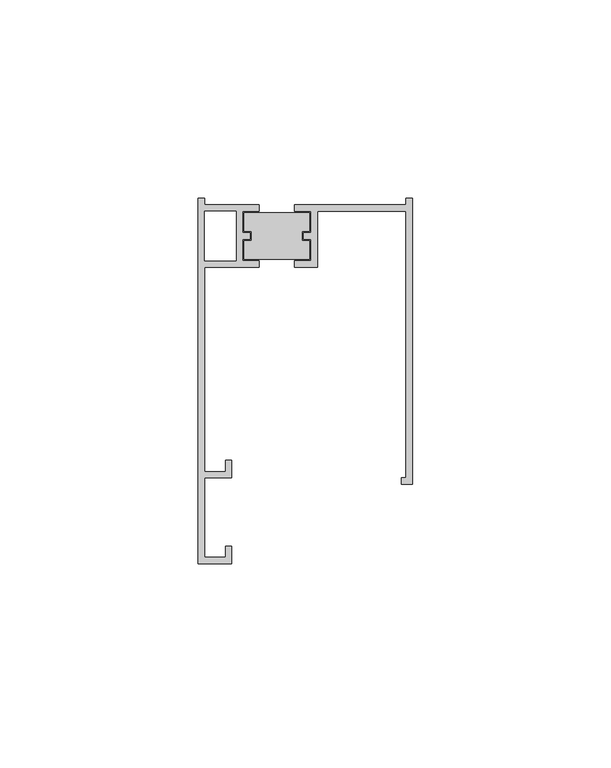
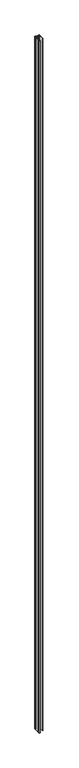
"""IFC4 building model written with IfcOpenShell, lengths in millimetres: proxy geometry, Generic Models 2:Generic Models 2:310765:Generic Models 2:310765 : Generic Models 2:Generic Models 2:310765:15 : Generic Models 2:Generic Models 2:310765:Generic Models 2:310765 : Generic Models 2:Generic Models 2:310765:300385."""

from ifc_helpers import new_model, si_unit, origin, origin_with_axes, place, context, project, spatial, polyline, outline, extrude, source, transform, mapped, element, save


def generic_models_0c4f637a(model_context):
    return source(origin(), model_context, "Body", "SweptSolid", [
        extrude(outline(polyline([(667633.5969099, -670386.8274693), (667617.0446537, -670386.8274693), (667617.0446537, -670382.1299707), (667618.9700691, -670382.1299707), (667618.9700691, -670379.7487207), (667617.0446537, -670379.7487207), (667617.0446537, -670375.0512221), (667633.5969099, -670375.0512221), (667633.5969099, -670379.7487207), (667631.6714944, -670379.7487207), (667631.6714944, -670382.1299707), (667633.5969099, -670382.1299707), (667633.5969099, -670386.8274693)])), origin_with_axes(), (0.0, 0.0, 1.0), 8775.8734497),
        extrude(outline(polyline([(667613.9760152, -670463.4793471), (667605.5296437, -670463.4793471), (667605.5296437, -670371.4793471), (667607.1171437, -670371.4793471), (667607.1171437, -670373.0668471), (667620.8149662, -670373.0668471), (667620.8149662, -670374.6543471), (667616.6477787, -670374.6543471), (667616.6477787, -670380.1455957), (667618.5731941, -670380.1455957), (667618.5731941, -670381.7330957), (667616.6477787, -670381.7330957), (667616.6477787, -670387.2243443), (667620.8149662, -670387.2243443), (667620.8149662, -670388.8118443), (667607.1171437, -670388.8118443), (667607.1171437, -670440.3043471), (667612.3885152, -670440.3043471), (667612.3885152, -670437.5045205), (667613.9760152, -670437.5045205), (667613.9760152, -670441.8918471), (667607.1171437, -670441.8918471), (667607.1171437, -670461.8918471), (667612.3885152, -670461.8918471), (667612.3885152, -670459.0920205), (667613.9760152, -670459.0920205), (667613.9760152, -670463.4793471)]), holes=[polyline([(667607.1171437, -670387.2243443), (667615.0602787, -670387.2243443), (667615.0602787, -670374.6543471), (667607.1171437, -670374.6543471), (667607.1171437, -670387.2243443)])]), origin_with_axes(), (0.0, 0.0, 1.0), 8775.8734497),
        extrude(outline(polyline([(667657.9421437, -670371.4793471), (667659.5296437, -670371.4793471), (667659.5296437, -670443.4793471), (667656.8145537, -670443.4793471), (667656.8145537, -670441.8918471), (667657.9421437, -670441.8918471), (667657.9421437, -670374.6543471), (667635.5812849, -670374.6543471), (667635.5812849, -670388.8118443), (667629.8265974, -670388.8118443), (667629.8265974, -670387.2243443), (667633.9937849, -670387.2243443), (667633.9937849, -670381.7330957), (667632.0683694, -670381.7330957), (667632.0683694, -670380.1455957), (667633.9937849, -670380.1455957), (667633.9937849, -670374.6543471), (667629.8265974, -670374.6543471), (667629.8265974, -670373.0668471), (667657.9421437, -670373.0668471), (667657.9421437, -670371.4793471)])), origin_with_axes(), (0.0, 0.0, 1.0), 8775.8734497),
    ])


if __name__ == "__main__":
    model = new_model("IFC4")
    model_context = context("Model", 3, world=origin())
    ifc_project = project(units=[si_unit("LENGTHUNIT", "METRE", prefix="MILLI")], contexts=[model_context])
    site = spatial("IfcSite", under=ifc_project)
    building = spatial("IfcBuilding", under=site)
    placement = place(None, origin())
    generic_models_shape = generic_models_0c4f637a(model_context)
    element("IfcBuildingElementProxy", 1, Name="Generic Models 2:Generic Models 2:310765:Generic Models 2:310765 : Generic Models 2:Generic Models 2:310765:15 : Generic Models 2:Generic Models 2:310765:Generic Models 2:310765 : Generic Models 2:Generic Models 2:310765:300385", ObjectType="Generic Models 2:Generic Models 2:310765:Generic Models 2:310765 : Generic Models 2:Generic Models 2:310765:15 : Generic Models 2:Generic Models 2:310765:Generic Models 2:310765 : Generic Models 2:Generic Models 2:310765:300385", at=placement, inside=building, context=model_context, shape_type="MappedRepresentation", body=[
        mapped(generic_models_shape, transform((0.0, 0.0, 0.0), x_axis=(1.0, 0.0, 0.0), y_axis=(0.0, 1.0, 0.0), z_axis=(0.0, 0.0, 1.0))),
    ])
    save(model, "model.ifc")

# Revit data of these elements
# Type "Generic Models 2:Generic Models 2:310765:Generic Models 2:310765 : Generic Models 2:Generic Models 2:310765:15 : Generic Models 2:Generic Models 2:310765:Generic Models 2:310765 : Generic Models 2:Generic Models 2:310765:300385"
#   NameOverride = "Generic Models 2:Generic Models 2:310765:Generic Models 2:310765 : Generic Models 2:Generic Models 2:310765:300385"
#   ObjectTypeOverride = "Generic Models 2:310765 : Generic Models 2:Generic Models 2:310765"
#   Reference = "Generic Models 2"
#   Tag = "300385"
# Element 1 (IfcBuildingElementProxy, "Generic Models 2:Generic Models 2:310765:Generic Models 2:310765 : Generic Models 2:Generic Models 2:310765:15 : Generic Models 2:Generic Models 2:310765:Generic Models 2:310765 : Generic Models 2:Generic Models 2:310765:300385")
#   Materials on its faces: "THERMAL BROKEN ALUMINUM STOREFRONT FOR POLYCARBONATE"
# Materials
#   "THERMAL BROKEN ALUMINUM STOREFRONT FOR POLYCARBONATE": class "Unassigned", colour RGB 244 244 244, transparency 0, Keynote = "M07611300.01", Cost = 0
